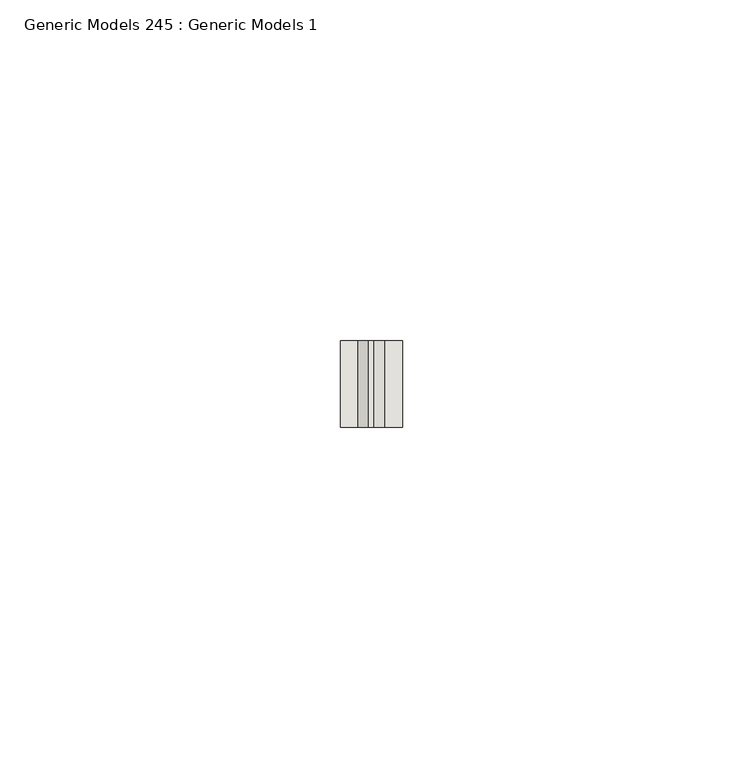
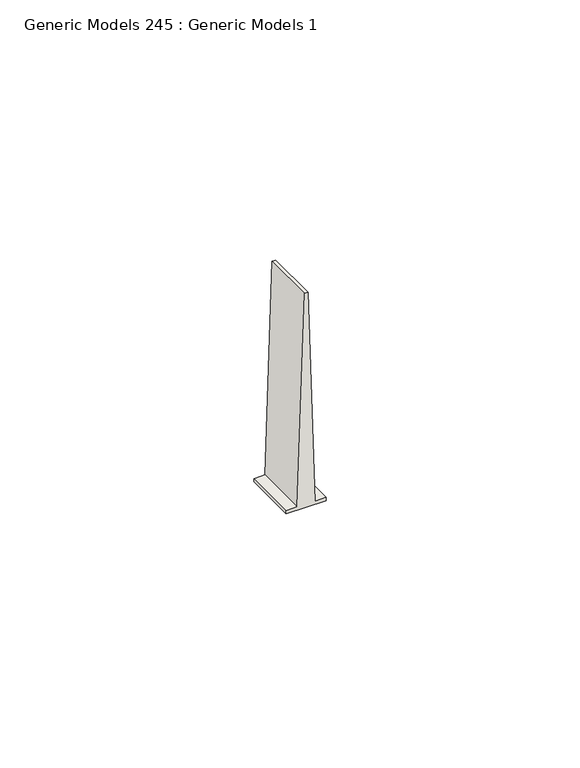
"""IFC4 building model written with IfcOpenShell, lengths in millimetres: wall geometry, Generic Models 245 : Generic Models 1."""

from ifc_helpers import new_model, si_unit, frame, origin, place, context, project, spatial, polyline, outline, extrude, source, transform, mapped, element, save


def generic_models_245_generic_models_1_1f39ab1d(model_context):
    return source(origin(), model_context, "Body", "SweptSolid", [
        extrude(outline(polyline([(5466.55625, 49733.4159), (5466.55625, 49742.5091), (5467.35, 49742.5091), (5467.35, 49739.9592364), (5518.15, 49738.3618473), (5518.15, 49737.5631527), (5467.35, 49735.9657636), (5467.35, 49733.4159), (5466.55625, 49733.4159)])), frame((0.0, 565.15, 0.0), z_axis=(0.0, 1.0, 0.0), x_axis=(0.0, 0.0, 1.0)), (0.0, 0.0, 1.0), 12.7),
    ])


if __name__ == "__main__":
    model = new_model("IFC4")
    model_context = context("Model", 3, world=origin())
    ifc_project = project(units=[si_unit("LENGTHUNIT", "METRE", prefix="MILLI")], contexts=[model_context])
    site = spatial("IfcSite", under=ifc_project)
    building = spatial("IfcBuilding", under=site)
    placement = place(None, origin())
    generic_models_245_generic_models_1_shape = generic_models_245_generic_models_1_1f39ab1d(model_context)
    element("IfcWall", 1, ObjectType="Generic Models 245 : Generic Models 1", at=placement, inside=building, context=model_context, shape_type="MappedRepresentation", body=[
        mapped(generic_models_245_generic_models_1_shape, transform((0.0, 0.0, 0.0), x_axis=(1.0, 0.0, 0.0), y_axis=(0.0, 1.0, 0.0), z_axis=(0.0, 0.0, 1.0))),
    ])
    save(model, "model.ifc")

# Revit data of these elements
# Element 1 (IfcWall, "Generic Models 245 : Generic Models 1")
#   Materials on its faces: "METAL RUNNER CHANNEL; FASTEN @ 24\" O.C."
# Materials
#   "METAL RUNNER CHANNEL; FASTEN @ 24\" O.C.": class "Unassigned", colour RGB 210 209 208, transparency 0, Keynote = "M05121300.02", Cost = 0
